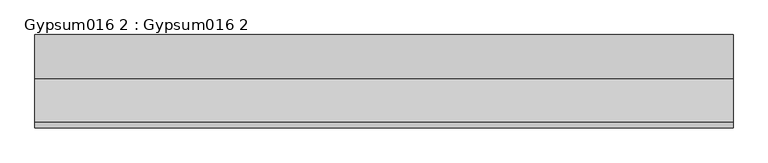
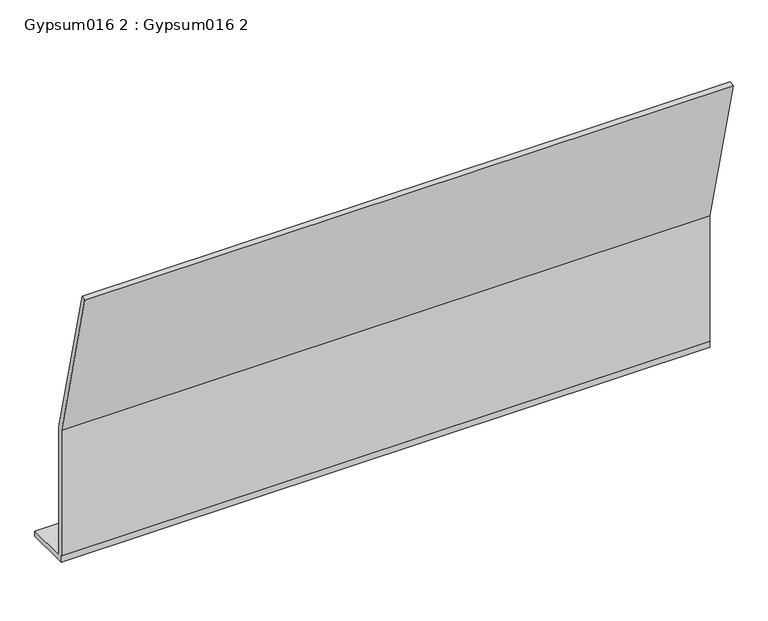
"""IFC4 building model written with IfcOpenShell, lengths in millimetres: proxy geometry, Gypsum016 2 : Gypsum016 2."""

from ifc_helpers import new_model, si_unit, frame, origin, place, context, project, spatial, polyline, outline, extrude, source, transform, mapped, element, save


def gypsum016_2_gypsum016_2_12ec1e8b(model_context):
    return source(origin(), model_context, "Body", "SweptSolid", [
        extrude(outline(polyline([(10278.0250834, 42906.696), (10404.7574604, 42906.696), (10404.7574604, 42890.821), (10284.5832673, 42890.821), (10284.5832673, 42892.101), (10263.4300834, 42892.101), (10263.4300834, 42913.2541839), (10262.1500834, 42913.2541839), (10262.1500834, 43322.8477886), (10137.3940009, 43821.8721184), (10152.7950131, 43825.7223714), (10278.0250834, 43324.8020904), (10278.0250834, 42906.696)])), frame((3694.2883192, 0.0, 0.0), z_axis=(1.0, 0.0, 0.0), x_axis=(0.0, 1.0, 0.0)), (0.0, 0.0, 1.0), 2000.0),
    ])


if __name__ == "__main__":
    model = new_model("IFC4")
    model_context = context("Model", 3, world=origin())
    ifc_project = project(units=[si_unit("LENGTHUNIT", "METRE", prefix="MILLI")], contexts=[model_context])
    site = spatial("IfcSite", under=ifc_project)
    building = spatial("IfcBuilding", under=site)
    placement = place(None, origin())
    gypsum016_2_gypsum016_2_shape = gypsum016_2_gypsum016_2_12ec1e8b(model_context)
    element("IfcBuildingElementProxy", 1, Name="Gypsum016 2 : Gypsum016 2", ObjectType="Gypsum016 2 : Gypsum016 2", at=placement, inside=building, context=model_context, shape_type="MappedRepresentation", body=[
        mapped(gypsum016_2_gypsum016_2_shape, transform((0.0, 0.0, 0.0), x_axis=(1.0, 0.0, 0.0), y_axis=(0.0, 1.0, 0.0), z_axis=(0.0, 0.0, 1.0))),
    ])
    save(model, "model.ifc")

# Revit data of these elements
# Type "Gypsum016 2 : Gypsum016 2"
#   NameOverride = "Gypsum016"
# Element 1 (IfcBuildingElementProxy, "Gypsum016 2 : Gypsum016 2")
#   Materials on its faces: "5/8\"  GYPSUM BOARD"
# Materials
#   "5/8\"  GYPSUM BOARD": class "Unassigned", colour RGB 255 255 255, transparency 0, Cost = 0
